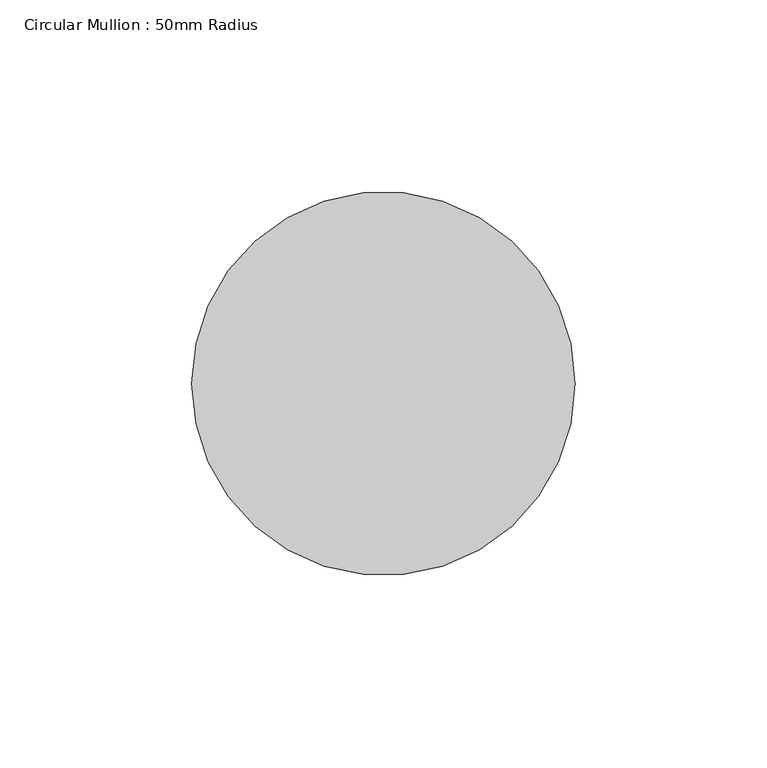
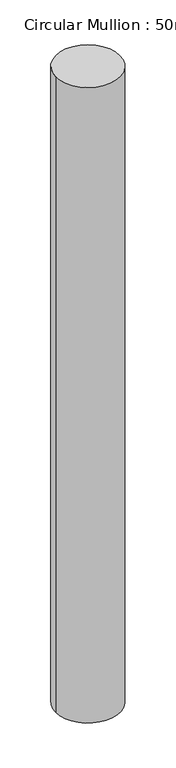
"""IFC4 building model written with IfcOpenShell, lengths in millimetres: member geometry, Circular Mullion : 50mm Radius."""

import ifcopenshell
import ifcopenshell.guid

model = None  # the IFC model being written
_history = None  # IfcOwnerHistory: only IFC2X3 demands one
_inside = {}  # id of a spatial element -> (the spatial element, [elements in it])
_under = {}  # id of a project, library or spatial element -> (it, [spatial elements below it])
_declared = {}  # id of a project -> (the project, [libraries it declares])
_typed = {}  # id of a type object -> (the type object, [elements of that type])
_made_of = {}  # id of a material, layer set ... -> (it, [elements and type objects made of it])


def new_model(schema):
    """Start an empty IFC model of exactly this schema.

    Asked for "IFC4X3", IfcOpenShell would pick the latest addendum, in which some entities
    have other attributes; the version numbers below select the first issue.
    IFC2X3 requires an IfcOwnerHistory on every rooted entity: one is made here for all.
    """
    global model, _history
    if schema == "IFC4X3":
        model = ifcopenshell.file(schema_version=(4, 3, 0, 0))
    else:
        model = ifcopenshell.file(schema=schema)
    _inside.clear()
    _under.clear()
    _declared.clear()
    _typed.clear()
    _made_of.clear()
    _history = None
    if model.schema == "IFC2X3":
        org = make("IfcOrganization", Name="unknown")
        user = make(
            "IfcPersonAndOrganization",
            ThePerson=make("IfcPerson", FamilyName="unknown"),
            TheOrganization=org,
        )
        app = make(
            "IfcApplication",
            ApplicationDeveloper=org,
            Version="unknown",
            ApplicationFullName="unknown",
            ApplicationIdentifier="unknown",
        )
        _history = make(
            "IfcOwnerHistory",
            OwningUser=user,
            OwningApplication=app,
            ChangeAction="ADDED",
            CreationDate=0,
        )
    return model


def make(cls, **values):
    """One entity of the class cls with the attributes given. An attribute that is None is left unset."""
    return model.create_entity(
        cls, **{name: value for name, value in values.items() if value is not None}
    )


def rooted(cls, **values):
    """An entity with a GlobalId (a new one), such as an element, a storey or a relation."""
    return make(cls, GlobalId=ifcopenshell.guid.new(), OwnerHistory=_history, **values)


def si_unit(unit_type, name, prefix=None):
    """IfcSIUnit, for example si_unit("LENGTHUNIT", "METRE", prefix="MILLI")."""
    return make("IfcSIUnit", UnitType=unit_type, Prefix=prefix, Name=name)


def assignment(units):
    """IfcUnitAssignment: the units of a project."""
    return None if units is None else make("IfcUnitAssignment", Units=units)


def point(xyz):
    """IfcCartesianPoint."""
    return None if xyz is None else make("IfcCartesianPoint", Coordinates=xyz)


def direction(xyz):
    """IfcDirection."""
    return None if xyz is None else make("IfcDirection", DirectionRatios=xyz)


def frame(location, z_axis=None, x_axis=None):
    """IfcAxis2Placement3D, a coordinate frame: its origin and axes. An axis left out is left unset."""
    return make(
        "IfcAxis2Placement3D",
        Location=point(location),
        Axis=direction(z_axis),
        RefDirection=direction(x_axis),
    )


def frame_2d(location, x_axis=None):
    """IfcAxis2Placement2D, a coordinate frame in the plane: its origin and x axis."""
    return make(
        "IfcAxis2Placement2D", Location=point(location), RefDirection=direction(x_axis)
    )


def origin():
    """The frame at (0, 0, 0) with its axes left unset."""
    return frame((0.0, 0.0, 0.0))


def origin_2d():
    """The frame at (0, 0) in the plane with its x axis left unset."""
    return frame_2d((0.0, 0.0))


def place(relative_to, where):
    """IfcLocalPlacement: puts the frame where relative to a parent placement (None: the world)."""
    return make(
        "IfcLocalPlacement", PlacementRelTo=relative_to, RelativePlacement=where
    )


def context(
    kind, dimensions, precision=None, world=None, true_north=None, identifier=None
):
    """IfcGeometricRepresentationContext, for example the 3D "Model" context."""
    return make(
        "IfcGeometricRepresentationContext",
        ContextIdentifier=identifier,
        ContextType=kind,
        CoordinateSpaceDimension=dimensions,
        Precision=precision,
        WorldCoordinateSystem=world,
        TrueNorth=true_north,
    )


def project(units=None, contexts=None):
    """IfcProject with its units and contexts."""
    return rooted(
        "IfcProject",
        Name="project",
        RepresentationContexts=contexts,
        UnitsInContext=assignment(units),
    )


def spatial(cls, under=None, at=None, **own):
    """A site, building, storey or space (cls), placed at a placement, below another one or the project."""
    s = rooted(cls, ObjectPlacement=at, **own)
    if under is not None:
        _under.setdefault(under.id(), (under, []))[1].append(s)
    return s


def circle_curve(where, radius):
    """IfcCircle in the frame where."""
    return make("IfcCircle", Position=where, Radius=radius)


def trimmed(basis, trim1, trim2, sense, master):
    """IfcTrimmedCurve: the piece of a basis curve between two trims."""
    return make(
        "IfcTrimmedCurve",
        BasisCurve=basis,
        Trim1=trim1,
        Trim2=trim2,
        SenseAgreement=sense,
        MasterRepresentation=master,
    )


def segment(curve, same_sense, transition):
    """IfcCompositeCurveSegment."""
    return make(
        "IfcCompositeCurveSegment",
        Transition=transition,
        SameSense=same_sense,
        ParentCurve=curve,
    )


def composite_curve(segments, self_intersect=None):
    """IfcCompositeCurve: segments joined end to end."""
    return make("IfcCompositeCurve", Segments=segments, SelfIntersect=self_intersect)


def outline(outer, holes=None, kind="AREA"):
    """IfcArbitraryClosedProfileDef: a profile drawn as a closed curve; with holes, ...WithVoids."""
    if holes is None:
        return make("IfcArbitraryClosedProfileDef", ProfileType=kind, OuterCurve=outer)
    return make(
        "IfcArbitraryProfileDefWithVoids",
        ProfileType=kind,
        OuterCurve=outer,
        InnerCurves=holes,
    )


def extrude(swept, where, along, depth):
    """IfcExtrudedAreaSolid: the profile swept, set in the frame where, extruded along a direction by depth."""
    return make(
        "IfcExtrudedAreaSolid",
        SweptArea=swept,
        Position=where,
        ExtrudedDirection=direction(along),
        Depth=depth,
    )


def shape(context_of_items, identifier, shape_type, items):
    """IfcShapeRepresentation: the items that make up one representation, for example the "Body"."""
    return make(
        "IfcShapeRepresentation",
        ContextOfItems=context_of_items,
        RepresentationIdentifier=identifier,
        RepresentationType=shape_type,
        Items=items,
    )


def source(mapping_origin, context_of_items, identifier, shape_type, items):
    """IfcRepresentationMap: a shape defined once, which mapped items show again and again."""
    return make(
        "IfcRepresentationMap",
        MappingOrigin=mapping_origin,
        MappedRepresentation=shape(context_of_items, identifier, shape_type, items),
    )


def transform(
    local_origin,
    x_axis=None,
    y_axis=None,
    z_axis=None,
    scale=None,
    scale2=None,
    scale3=None,
    uniform=True,
):
    """IfcCartesianTransformationOperator3D, or its non-uniform kind. x_axis, y_axis, z_axis: its Axis1, 2, 3."""
    if uniform:
        return make(
            "IfcCartesianTransformationOperator3D",
            Axis1=direction(x_axis),
            Axis2=direction(y_axis),
            LocalOrigin=point(local_origin),
            Scale=scale,
            Axis3=direction(z_axis),
        )
    return make(
        "IfcCartesianTransformationOperator3DnonUniform",
        Axis1=direction(x_axis),
        Axis2=direction(y_axis),
        LocalOrigin=point(local_origin),
        Scale=scale,
        Axis3=direction(z_axis),
        Scale2=scale2,
        Scale3=scale3,
    )


def mapped(mapping_source, mapping_target):
    """IfcMappedItem: shows the shape of a source again, moved by a transform."""
    return make(
        "IfcMappedItem", MappingSource=mapping_source, MappingTarget=mapping_target
    )


def made_of(thing, what):
    """Note that an element or type object is made of a material, layer set ...; save() writes the relation."""
    if what is not None:
        _made_of.setdefault(what.id(), (what, []))[1].append(thing)
    return thing


def element(
    cls,
    number,
    at=None,
    inside=None,
    cuts=None,
    type_object=None,
    material=None,
    context=None,
    identifier="Body",
    shape_type=None,
    held_by="IfcProductDefinitionShape",
    body=None,
    shapes=None,
    **own,
):
    """One element of the class cls, such as IfcWall. Its Tag is "e" and its number.

    at: its placement. inside: the storey or other place that contains it. cuts: it is an
    opening in that element (IfcRelVoidsElement). A single representation is given by context,
    identifier, shape_type and body (its items); several are given by shapes. held_by: the class
    of the entity that holds the representations. save() writes the other relations.
    """
    e = rooted(cls, Tag="e%d" % number, ObjectPlacement=at, **own)
    if body is not None:
        shapes = [shape(context, identifier, shape_type, body)]
    if shapes is not None:
        e.Representation = make(held_by, Representations=shapes)
    if inside is not None:
        _inside.setdefault(inside.id(), (inside, []))[1].append(e)
    if cuts is not None:
        rooted(
            "IfcRelVoidsElement", RelatingBuildingElement=cuts, RelatedOpeningElement=e
        )
    if type_object is not None:
        _typed.setdefault(type_object.id(), (type_object, []))[1].append(e)
    return made_of(e, material)


def aggregate(whole, parts):
    """IfcRelAggregates: a whole, such as a stair, and the parts it consists of."""
    return rooted("IfcRelAggregates", RelatingObject=whole, RelatedObjects=parts)


def save(model, path):
    """Write the relations noted so far, then the file.

    IfcRelAggregates (storeys below a building ...), IfcRelContainedInSpatialStructure (elements
    in a storey), IfcRelDefinesByType, IfcRelAssociatesMaterial and IfcRelDeclares: one each for
    every whole, place, type object, material and project.
    """
    for whole, parts in _under.values():
        aggregate(whole, parts)
    for where, things in _inside.values():
        rooted(
            "IfcRelContainedInSpatialStructure",
            RelatedElements=things,
            RelatingStructure=where,
        )
    for kind, things in _typed.values():
        rooted("IfcRelDefinesByType", RelatedObjects=things, RelatingType=kind)
    for what, things in _made_of.values():
        rooted("IfcRelAssociatesMaterial", RelatedObjects=things, RelatingMaterial=what)
    for by, libraries in _declared.values():
        rooted("IfcRelDeclares", RelatingContext=by, RelatedDefinitions=libraries)
    model.write(path)


def circular_mullion_50mm_radius_970eb5e9(model_context):
    return source(origin(), model_context, "Body", "SweptSolid", [
        extrude(outline(composite_curve([segment(trimmed(circle_curve(origin_2d(), 50.0), [point((50.0, 0.0))], [point((-50.0, 0.0))], False, "CARTESIAN"), True, "CONTINUOUS"), segment(trimmed(circle_curve(origin_2d(), 50.0), [point((-50.0, 0.0))], [point((50.0, 0.0))], False, "CARTESIAN"), True, "CONTINUOUS")], self_intersect=False)), frame((0.0, 0.0, -1045.4844762), z_axis=(0.0, 0.0, 1.0), x_axis=(1.0, 0.0, 0.0)), (0.0, 0.0, 1.0), 1045.4844762),
    ])


if __name__ == "__main__":
    model = new_model("IFC4")
    model_context = context("Model", 3, world=origin())
    ifc_project = project(units=[si_unit("LENGTHUNIT", "METRE", prefix="MILLI")], contexts=[model_context])
    site = spatial("IfcSite", under=ifc_project)
    building = spatial("IfcBuilding", under=site)
    placement = place(None, origin())
    circular_mullion_50mm_radius_shape = circular_mullion_50mm_radius_970eb5e9(model_context)
    element("IfcMember", 1, ObjectType="Circular Mullion : 50mm Radius", at=placement, inside=building, context=model_context, shape_type="MappedRepresentation", body=[
        mapped(circular_mullion_50mm_radius_shape, transform((0.0, 0.0, 0.0), x_axis=(1.0, 0.0, 0.0), y_axis=(0.0, 1.0, 0.0), z_axis=(0.0, 0.0, 1.0))),
    ])
    save(model, "model.ifc")

# Revit data of these elements
# Type "Circular Mullion : 50mm Radius"
#   built-in parameter 1007350 = 0.164042 (stored number, unit not read)
# Element 1 (IfcMember, "Circular Mullion : 50mm Radius")
#   Materials on its faces: "Aluminium"
# Materials
#   "Aluminium": class "Metal", colour RGB 247 247 247, transparency 0, Description = "Aluminium 6061", Cost = 0
